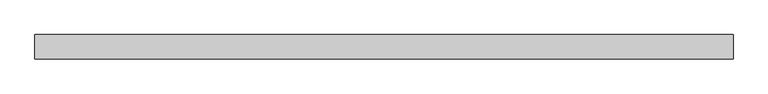
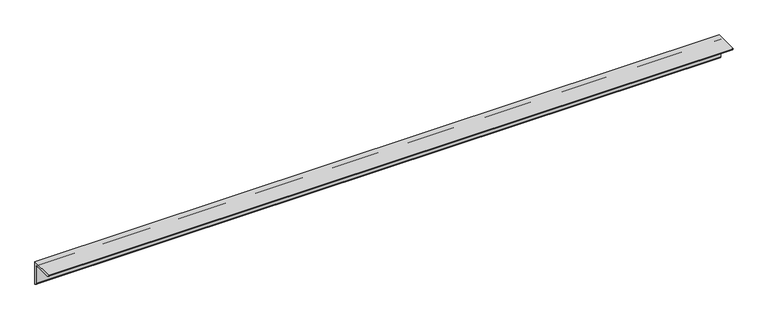
"""IFC4 building model written with IfcOpenShell, lengths in millimetres: member geometry, 0912_Steel Framing_L-KSD3502 : H_SB_AR_S03_L-130x130x12_HBR3."""

from ifc_helpers import new_model, si_unit, point, frame, frame_2d, origin, place, context, project, spatial, polyline, circle_curve, trimmed, segment, composite_curve, outline, extrude, source, transform, mapped, element, save


def member_26543d8b(model_context):
    return source(origin(), model_context, "Body", "SweptSolid", [
        extrude(outline(composite_curve([segment(polyline([(36.4, 36.4), (36.4, -93.6)]), True, "CONTINUOUS"), segment(trimmed(circle_curve(frame_2d((36.4, -81.6)), 12.0), [point((36.4, -93.6))], [point((24.4, -81.6))], False, "CARTESIAN"), True, "CONTINUOUS"), segment(polyline([(24.4, -81.6), (24.4, 12.4)]), True, "CONTINUOUS"), segment(trimmed(circle_curve(frame_2d((12.4, 12.4)), 12.0), [point((24.4, 12.4))], [point((12.4, 24.4))], True, "CARTESIAN"), True, "CONTINUOUS"), segment(polyline([(12.4, 24.4), (-81.6, 24.4)]), True, "CONTINUOUS"), segment(trimmed(circle_curve(frame_2d((-81.6, 36.4)), 12.0), [point((-81.6, 24.4))], [point((-93.6, 36.4))], False, "CARTESIAN"), True, "CONTINUOUS"), segment(polyline([(-93.6, 36.4), (36.4, 36.4)]), True, "CONTINUOUS")], self_intersect=False)), frame((-1903.5603013, 0.0, 0.0), z_axis=(1.0, 0.0, 0.0), x_axis=(0.0, 1.0, 0.0)), (0.0, 0.0, 1.0), 3729.3286027),
    ])


if __name__ == "__main__":
    model = new_model("IFC4")
    model_context = context("Model", 3, world=origin())
    ifc_project = project(units=[si_unit("LENGTHUNIT", "METRE", prefix="MILLI")], contexts=[model_context])
    site = spatial("IfcSite", under=ifc_project)
    building = spatial("IfcBuilding", under=site)
    placement = place(None, origin())
    member_shape = member_26543d8b(model_context)
    element("IfcMember", 1, ObjectType="0912_Steel Framing_L-KSD3502 : H_SB_AR_S03_L-130x130x12_HBR3", at=placement, inside=building, context=model_context, shape_type="MappedRepresentation", body=[
        mapped(member_shape, transform((0.0, 0.0, 0.0), x_axis=(1.0, 0.0, 0.0), y_axis=(0.0, 1.0, 0.0), z_axis=(0.0, 0.0, 1.0))),
    ])
    save(model, "model.ifc")

# Revit data of these elements
# Type "0912_Steel Framing_L-KSD3502 : H_SB_AR_S03_L-130x130x12_HBR3"
#   k = 25 mm
#   Perimeter = 0.52 m²/m
#   Nominal Weight = 23.40 kgf/m
#   Length [instance default] = 1000 mm
#   b = 130 mm
#   d = 130 mm
#   t = 12 mm
#   x = 36.4 mm
#   y = 36.4 mm
#   A = 2976.00 m²
#   Structural Material [instance default] = Steel, 45-345
# Element 1 (IfcMember, "0912_Steel Framing_L-KSD3502 : H_SB_AR_S03_L-130x130x12_HBR3")
#   Structural Material = Steel ASTM A36
#   Materials on its faces: "Steel ASTM A36"
# Materials
#   "Steel, 45-345": class "Metal", colour RGB 189 187 185, transparency 0, Description = "Steel 345 MPa", Cost = 0
#   "Steel ASTM A36": class "Metal", colour RGB 199 199 199, transparency 0, Description = "Structural steel, ASTM A36 Grade B, mill finish", Cost = 0
